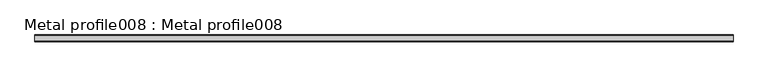
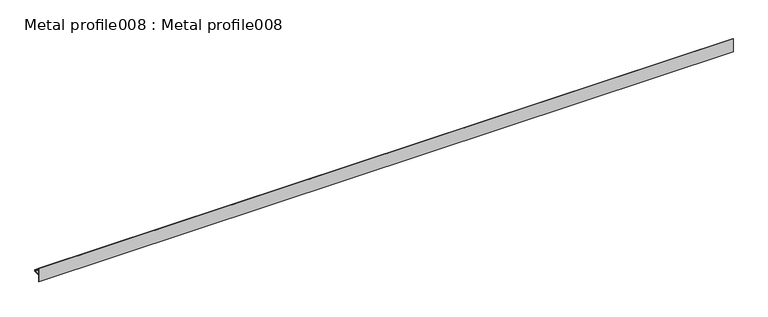
"""IFC4 building model written with IfcOpenShell, lengths in millimetres: proxy geometry, Metal profile008 : Metal profile008."""

import ifcopenshell
import ifcopenshell.guid

model = None  # the IFC model being written
_history = None  # IfcOwnerHistory: only IFC2X3 demands one
_inside = {}  # id of a spatial element -> (the spatial element, [elements in it])
_under = {}  # id of a project, library or spatial element -> (it, [spatial elements below it])
_declared = {}  # id of a project -> (the project, [libraries it declares])
_typed = {}  # id of a type object -> (the type object, [elements of that type])
_made_of = {}  # id of a material, layer set ... -> (it, [elements and type objects made of it])


def new_model(schema):
    """Start an empty IFC model of exactly this schema.

    Asked for "IFC4X3", IfcOpenShell would pick the latest addendum, in which some entities
    have other attributes; the version numbers below select the first issue.
    IFC2X3 requires an IfcOwnerHistory on every rooted entity: one is made here for all.
    """
    global model, _history
    if schema == "IFC4X3":
        model = ifcopenshell.file(schema_version=(4, 3, 0, 0))
    else:
        model = ifcopenshell.file(schema=schema)
    _inside.clear()
    _under.clear()
    _declared.clear()
    _typed.clear()
    _made_of.clear()
    _history = None
    if model.schema == "IFC2X3":
        org = make("IfcOrganization", Name="unknown")
        user = make(
            "IfcPersonAndOrganization",
            ThePerson=make("IfcPerson", FamilyName="unknown"),
            TheOrganization=org,
        )
        app = make(
            "IfcApplication",
            ApplicationDeveloper=org,
            Version="unknown",
            ApplicationFullName="unknown",
            ApplicationIdentifier="unknown",
        )
        _history = make(
            "IfcOwnerHistory",
            OwningUser=user,
            OwningApplication=app,
            ChangeAction="ADDED",
            CreationDate=0,
        )
    return model


def make(cls, **values):
    """One entity of the class cls with the attributes given. An attribute that is None is left unset."""
    return model.create_entity(
        cls, **{name: value for name, value in values.items() if value is not None}
    )


def rooted(cls, **values):
    """An entity with a GlobalId (a new one), such as an element, a storey or a relation."""
    return make(cls, GlobalId=ifcopenshell.guid.new(), OwnerHistory=_history, **values)


def si_unit(unit_type, name, prefix=None):
    """IfcSIUnit, for example si_unit("LENGTHUNIT", "METRE", prefix="MILLI")."""
    return make("IfcSIUnit", UnitType=unit_type, Prefix=prefix, Name=name)


def assignment(units):
    """IfcUnitAssignment: the units of a project."""
    return None if units is None else make("IfcUnitAssignment", Units=units)


def point(xyz):
    """IfcCartesianPoint."""
    return None if xyz is None else make("IfcCartesianPoint", Coordinates=xyz)


def direction(xyz):
    """IfcDirection."""
    return None if xyz is None else make("IfcDirection", DirectionRatios=xyz)


def frame(location, z_axis=None, x_axis=None):
    """IfcAxis2Placement3D, a coordinate frame: its origin and axes. An axis left out is left unset."""
    return make(
        "IfcAxis2Placement3D",
        Location=point(location),
        Axis=direction(z_axis),
        RefDirection=direction(x_axis),
    )


def origin():
    """The frame at (0, 0, 0) with its axes left unset."""
    return frame((0.0, 0.0, 0.0))


def place(relative_to, where):
    """IfcLocalPlacement: puts the frame where relative to a parent placement (None: the world)."""
    return make(
        "IfcLocalPlacement", PlacementRelTo=relative_to, RelativePlacement=where
    )


def context(
    kind, dimensions, precision=None, world=None, true_north=None, identifier=None
):
    """IfcGeometricRepresentationContext, for example the 3D "Model" context."""
    return make(
        "IfcGeometricRepresentationContext",
        ContextIdentifier=identifier,
        ContextType=kind,
        CoordinateSpaceDimension=dimensions,
        Precision=precision,
        WorldCoordinateSystem=world,
        TrueNorth=true_north,
    )


def project(units=None, contexts=None):
    """IfcProject with its units and contexts."""
    return rooted(
        "IfcProject",
        Name="project",
        RepresentationContexts=contexts,
        UnitsInContext=assignment(units),
    )


def spatial(cls, under=None, at=None, **own):
    """A site, building, storey or space (cls), placed at a placement, below another one or the project."""
    s = rooted(cls, ObjectPlacement=at, **own)
    if under is not None:
        _under.setdefault(under.id(), (under, []))[1].append(s)
    return s


def polyline(points):
    """IfcPolyline through the points."""
    return make("IfcPolyline", Points=[point(p) for p in points])


def outline(outer, holes=None, kind="AREA"):
    """IfcArbitraryClosedProfileDef: a profile drawn as a closed curve; with holes, ...WithVoids."""
    if holes is None:
        return make("IfcArbitraryClosedProfileDef", ProfileType=kind, OuterCurve=outer)
    return make(
        "IfcArbitraryProfileDefWithVoids",
        ProfileType=kind,
        OuterCurve=outer,
        InnerCurves=holes,
    )


def extrude(swept, where, along, depth):
    """IfcExtrudedAreaSolid: the profile swept, set in the frame where, extruded along a direction by depth."""
    return make(
        "IfcExtrudedAreaSolid",
        SweptArea=swept,
        Position=where,
        ExtrudedDirection=direction(along),
        Depth=depth,
    )


def shape(context_of_items, identifier, shape_type, items):
    """IfcShapeRepresentation: the items that make up one representation, for example the "Body"."""
    return make(
        "IfcShapeRepresentation",
        ContextOfItems=context_of_items,
        RepresentationIdentifier=identifier,
        RepresentationType=shape_type,
        Items=items,
    )


def source(mapping_origin, context_of_items, identifier, shape_type, items):
    """IfcRepresentationMap: a shape defined once, which mapped items show again and again."""
    return make(
        "IfcRepresentationMap",
        MappingOrigin=mapping_origin,
        MappedRepresentation=shape(context_of_items, identifier, shape_type, items),
    )


def transform(
    local_origin,
    x_axis=None,
    y_axis=None,
    z_axis=None,
    scale=None,
    scale2=None,
    scale3=None,
    uniform=True,
):
    """IfcCartesianTransformationOperator3D, or its non-uniform kind. x_axis, y_axis, z_axis: its Axis1, 2, 3."""
    if uniform:
        return make(
            "IfcCartesianTransformationOperator3D",
            Axis1=direction(x_axis),
            Axis2=direction(y_axis),
            LocalOrigin=point(local_origin),
            Scale=scale,
            Axis3=direction(z_axis),
        )
    return make(
        "IfcCartesianTransformationOperator3DnonUniform",
        Axis1=direction(x_axis),
        Axis2=direction(y_axis),
        LocalOrigin=point(local_origin),
        Scale=scale,
        Axis3=direction(z_axis),
        Scale2=scale2,
        Scale3=scale3,
    )


def mapped(mapping_source, mapping_target):
    """IfcMappedItem: shows the shape of a source again, moved by a transform."""
    return make(
        "IfcMappedItem", MappingSource=mapping_source, MappingTarget=mapping_target
    )


def made_of(thing, what):
    """Note that an element or type object is made of a material, layer set ...; save() writes the relation."""
    if what is not None:
        _made_of.setdefault(what.id(), (what, []))[1].append(thing)
    return thing


def element(
    cls,
    number,
    at=None,
    inside=None,
    cuts=None,
    type_object=None,
    material=None,
    context=None,
    identifier="Body",
    shape_type=None,
    held_by="IfcProductDefinitionShape",
    body=None,
    shapes=None,
    **own,
):
    """One element of the class cls, such as IfcWall. Its Tag is "e" and its number.

    at: its placement. inside: the storey or other place that contains it. cuts: it is an
    opening in that element (IfcRelVoidsElement). A single representation is given by context,
    identifier, shape_type and body (its items); several are given by shapes. held_by: the class
    of the entity that holds the representations. save() writes the other relations.
    """
    e = rooted(cls, Tag="e%d" % number, ObjectPlacement=at, **own)
    if body is not None:
        shapes = [shape(context, identifier, shape_type, body)]
    if shapes is not None:
        e.Representation = make(held_by, Representations=shapes)
    if inside is not None:
        _inside.setdefault(inside.id(), (inside, []))[1].append(e)
    if cuts is not None:
        rooted(
            "IfcRelVoidsElement", RelatingBuildingElement=cuts, RelatedOpeningElement=e
        )
    if type_object is not None:
        _typed.setdefault(type_object.id(), (type_object, []))[1].append(e)
    return made_of(e, material)


def aggregate(whole, parts):
    """IfcRelAggregates: a whole, such as a stair, and the parts it consists of."""
    return rooted("IfcRelAggregates", RelatingObject=whole, RelatedObjects=parts)


def save(model, path):
    """Write the relations noted so far, then the file.

    IfcRelAggregates (storeys below a building ...), IfcRelContainedInSpatialStructure (elements
    in a storey), IfcRelDefinesByType, IfcRelAssociatesMaterial and IfcRelDeclares: one each for
    every whole, place, type object, material and project.
    """
    for whole, parts in _under.values():
        aggregate(whole, parts)
    for where, things in _inside.values():
        rooted(
            "IfcRelContainedInSpatialStructure",
            RelatedElements=things,
            RelatingStructure=where,
        )
    for kind, things in _typed.values():
        rooted("IfcRelDefinesByType", RelatedObjects=things, RelatingType=kind)
    for what, things in _made_of.values():
        rooted("IfcRelAssociatesMaterial", RelatedObjects=things, RelatingMaterial=what)
    for by, libraries in _declared.values():
        rooted("IfcRelDeclares", RelatingContext=by, RelatedDefinitions=libraries)
    model.write(path)


def metal_profile008_metal_profile008_e2d48ebb(model_context):
    return source(origin(), model_context, "Body", "SweptSolid", [
        extrude(outline(polyline([(10466.6940287, 42935.1099451), (10466.6940287, 42930.3601451), (10448.4600807, 42930.3601451), (10448.4600807, 42911.3101451), (10447.1900807, 42911.3101451), (10447.1900807, 42950.6801451), (10448.4600807, 42950.6801451), (10448.4600807, 42931.6301451), (10465.4240287, 42931.6301451), (10465.4240287, 42935.1099451), (10466.6940287, 42935.1099451)])), frame((3694.2883192, 0.0, 0.0), z_axis=(1.0, 0.0, 0.0), x_axis=(0.0, 1.0, 0.0)), (0.0, 0.0, 1.0), 2000.0),
    ])


if __name__ == "__main__":
    model = new_model("IFC4")
    model_context = context("Model", 3, world=origin())
    ifc_project = project(units=[si_unit("LENGTHUNIT", "METRE", prefix="MILLI")], contexts=[model_context])
    site = spatial("IfcSite", under=ifc_project)
    building = spatial("IfcBuilding", under=site)
    placement = place(None, origin())
    metal_profile008_metal_profile008_shape = metal_profile008_metal_profile008_e2d48ebb(model_context)
    element("IfcBuildingElementProxy", 1, Name="Metal profile008 : Metal profile008", ObjectType="Metal profile008 : Metal profile008", at=placement, inside=building, context=model_context, shape_type="MappedRepresentation", body=[
        mapped(metal_profile008_metal_profile008_shape, transform((0.0, 0.0, 0.0), x_axis=(1.0, 0.0, 0.0), y_axis=(0.0, 1.0, 0.0), z_axis=(0.0, 0.0, 1.0))),
    ])
    save(model, "model.ifc")

# Revit data of these elements
# Type "Metal profile008 : Metal profile008"
#   NameOverride = "Metal profile008"
# Element 1 (IfcBuildingElementProxy, "Metal profile008 : Metal profile008")
#   Materials on its faces: "16 GA. COPPER VENTED T REVEAL BEAD"
# Materials
#   "16 GA. COPPER VENTED T REVEAL BEAD": class "Unassigned", colour RGB 255 227 10, transparency 0
